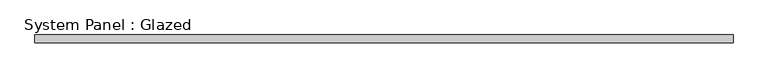
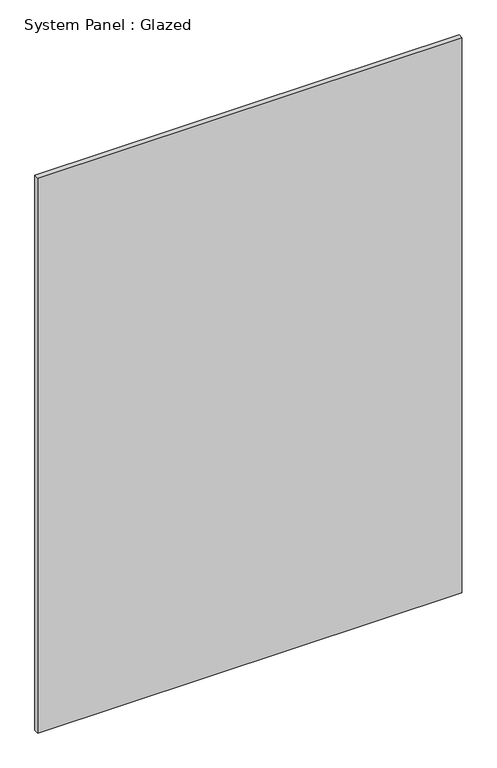
"""IFC4 building model written with IfcOpenShell, lengths in millimetres: plate geometry, System Panel : Glazed."""

from ifc_helpers import new_model, si_unit, origin, origin_with_axes, place, context, project, spatial, polyline, outline, extrude, source, transform, mapped, element, save


def system_panel_glazed_4d4608c9(model_context):
    return source(origin(), model_context, "Body", "SweptSolid", [
        extrude(outline(polyline([(1145.9716649, 24.5), (-1145.9716649, 24.5), (-1145.9716649, 49.5), (1145.9716649, 49.5), (1145.9716649, 24.5)])), origin_with_axes(), (0.0, 0.0, 1.0), 3170.0),
    ])


if __name__ == "__main__":
    model = new_model("IFC4")
    model_context = context("Model", 3, world=origin())
    ifc_project = project(units=[si_unit("LENGTHUNIT", "METRE", prefix="MILLI")], contexts=[model_context])
    site = spatial("IfcSite", under=ifc_project)
    building = spatial("IfcBuilding", under=site)
    placement = place(None, origin())
    system_panel_glazed_shape = system_panel_glazed_4d4608c9(model_context)
    element("IfcPlate", 1, ObjectType="System Panel : Glazed", at=placement, inside=building, context=model_context, shape_type="MappedRepresentation", body=[
        mapped(system_panel_glazed_shape, transform((0.0, 0.0, 0.0), x_axis=(1.0, 0.0, 0.0), y_axis=(0.0, 1.0, 0.0), z_axis=(0.0, 0.0, 1.0))),
    ])
    save(model, "model.ifc")

# Revit data of these elements
# Type "System Panel : Glazed"
#   Construction Type Id = "GSP4R"
#   Analytic Construction = "1/8 in Pilkington single glazing"
#   Visual Light Transmittance = 0.9
#   Solar Heat Gain Coefficient = 0.86
#   Heat Transfer Coefficient (U) = 6.7069 W/(m²·K)
#   Define Thermal Properties by = 1
# Element 1 (IfcPlate, "System Panel : Glazed")
#   Materials on its faces: "Glass"
# Materials
#   "Glass": class "Glass", colour RGB 245 245 243, transparency 1, Description = "Soda Lime Glass", Cost = 0
